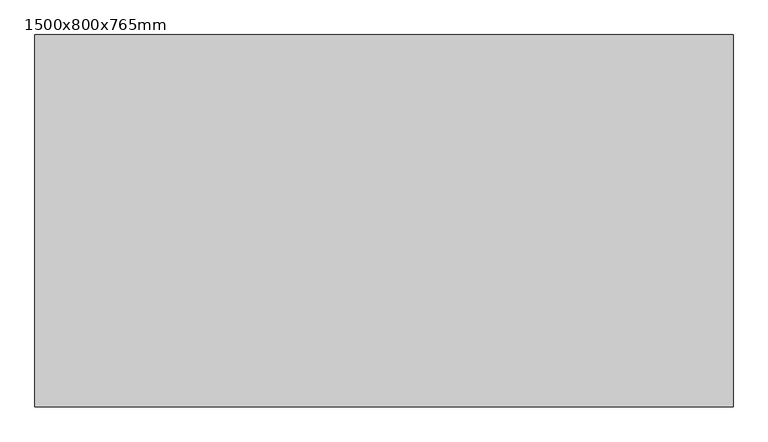
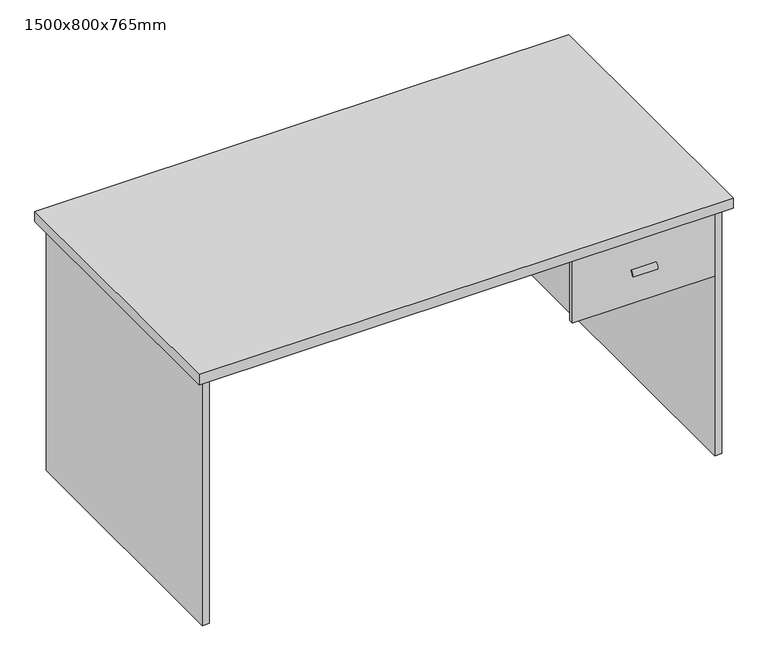
"""IFC4 building model written with IfcOpenShell, lengths in millimetres: furniture geometry, NBS_OffcDsks_OfficeDeskWithDrawer : 1500x800x765mm."""

import ifcopenshell
import ifcopenshell.guid

model = None  # the IFC model being written
_history = None  # IfcOwnerHistory: only IFC2X3 demands one
_inside = {}  # id of a spatial element -> (the spatial element, [elements in it])
_under = {}  # id of a project, library or spatial element -> (it, [spatial elements below it])
_declared = {}  # id of a project -> (the project, [libraries it declares])
_typed = {}  # id of a type object -> (the type object, [elements of that type])
_made_of = {}  # id of a material, layer set ... -> (it, [elements and type objects made of it])


def new_model(schema):
    """Start an empty IFC model of exactly this schema.

    Asked for "IFC4X3", IfcOpenShell would pick the latest addendum, in which some entities
    have other attributes; the version numbers below select the first issue.
    IFC2X3 requires an IfcOwnerHistory on every rooted entity: one is made here for all.
    """
    global model, _history
    if schema == "IFC4X3":
        model = ifcopenshell.file(schema_version=(4, 3, 0, 0))
    else:
        model = ifcopenshell.file(schema=schema)
    _inside.clear()
    _under.clear()
    _declared.clear()
    _typed.clear()
    _made_of.clear()
    _history = None
    if model.schema == "IFC2X3":
        org = make("IfcOrganization", Name="unknown")
        user = make(
            "IfcPersonAndOrganization",
            ThePerson=make("IfcPerson", FamilyName="unknown"),
            TheOrganization=org,
        )
        app = make(
            "IfcApplication",
            ApplicationDeveloper=org,
            Version="unknown",
            ApplicationFullName="unknown",
            ApplicationIdentifier="unknown",
        )
        _history = make(
            "IfcOwnerHistory",
            OwningUser=user,
            OwningApplication=app,
            ChangeAction="ADDED",
            CreationDate=0,
        )
    return model


def make(cls, **values):
    """One entity of the class cls with the attributes given. An attribute that is None is left unset."""
    return model.create_entity(
        cls, **{name: value for name, value in values.items() if value is not None}
    )


def rooted(cls, **values):
    """An entity with a GlobalId (a new one), such as an element, a storey or a relation."""
    return make(cls, GlobalId=ifcopenshell.guid.new(), OwnerHistory=_history, **values)


def si_unit(unit_type, name, prefix=None):
    """IfcSIUnit, for example si_unit("LENGTHUNIT", "METRE", prefix="MILLI")."""
    return make("IfcSIUnit", UnitType=unit_type, Prefix=prefix, Name=name)


def assignment(units):
    """IfcUnitAssignment: the units of a project."""
    return None if units is None else make("IfcUnitAssignment", Units=units)


def point(xyz):
    """IfcCartesianPoint."""
    return None if xyz is None else make("IfcCartesianPoint", Coordinates=xyz)


def direction(xyz):
    """IfcDirection."""
    return None if xyz is None else make("IfcDirection", DirectionRatios=xyz)


def frame(location, z_axis=None, x_axis=None):
    """IfcAxis2Placement3D, a coordinate frame: its origin and axes. An axis left out is left unset."""
    return make(
        "IfcAxis2Placement3D",
        Location=point(location),
        Axis=direction(z_axis),
        RefDirection=direction(x_axis),
    )


def frame_2d(location, x_axis=None):
    """IfcAxis2Placement2D, a coordinate frame in the plane: its origin and x axis."""
    return make(
        "IfcAxis2Placement2D", Location=point(location), RefDirection=direction(x_axis)
    )


def origin():
    """The frame at (0, 0, 0) with its axes left unset."""
    return frame((0.0, 0.0, 0.0))


def origin_with_axes():
    """The frame at (0, 0, 0) with the z axis (0, 0, 1) and the x axis (1, 0, 0) written out."""
    return frame((0.0, 0.0, 0.0), z_axis=(0.0, 0.0, 1.0), x_axis=(1.0, 0.0, 0.0))


def place(relative_to, where):
    """IfcLocalPlacement: puts the frame where relative to a parent placement (None: the world)."""
    return make(
        "IfcLocalPlacement", PlacementRelTo=relative_to, RelativePlacement=where
    )


def context(
    kind, dimensions, precision=None, world=None, true_north=None, identifier=None
):
    """IfcGeometricRepresentationContext, for example the 3D "Model" context."""
    return make(
        "IfcGeometricRepresentationContext",
        ContextIdentifier=identifier,
        ContextType=kind,
        CoordinateSpaceDimension=dimensions,
        Precision=precision,
        WorldCoordinateSystem=world,
        TrueNorth=true_north,
    )


def project(units=None, contexts=None):
    """IfcProject with its units and contexts."""
    return rooted(
        "IfcProject",
        Name="project",
        RepresentationContexts=contexts,
        UnitsInContext=assignment(units),
    )


def spatial(cls, under=None, at=None, **own):
    """A site, building, storey or space (cls), placed at a placement, below another one or the project."""
    s = rooted(cls, ObjectPlacement=at, **own)
    if under is not None:
        _under.setdefault(under.id(), (under, []))[1].append(s)
    return s


def polyline(points):
    """IfcPolyline through the points."""
    return make("IfcPolyline", Points=[point(p) for p in points])


def circle_curve(where, radius):
    """IfcCircle in the frame where."""
    return make("IfcCircle", Position=where, Radius=radius)


def trimmed(basis, trim1, trim2, sense, master):
    """IfcTrimmedCurve: the piece of a basis curve between two trims."""
    return make(
        "IfcTrimmedCurve",
        BasisCurve=basis,
        Trim1=trim1,
        Trim2=trim2,
        SenseAgreement=sense,
        MasterRepresentation=master,
    )


def segment(curve, same_sense, transition):
    """IfcCompositeCurveSegment."""
    return make(
        "IfcCompositeCurveSegment",
        Transition=transition,
        SameSense=same_sense,
        ParentCurve=curve,
    )


def composite_curve(segments, self_intersect=None):
    """IfcCompositeCurve: segments joined end to end."""
    return make("IfcCompositeCurve", Segments=segments, SelfIntersect=self_intersect)


def outline(outer, holes=None, kind="AREA"):
    """IfcArbitraryClosedProfileDef: a profile drawn as a closed curve; with holes, ...WithVoids."""
    if holes is None:
        return make("IfcArbitraryClosedProfileDef", ProfileType=kind, OuterCurve=outer)
    return make(
        "IfcArbitraryProfileDefWithVoids",
        ProfileType=kind,
        OuterCurve=outer,
        InnerCurves=holes,
    )


def extrude(swept, where, along, depth):
    """IfcExtrudedAreaSolid: the profile swept, set in the frame where, extruded along a direction by depth."""
    return make(
        "IfcExtrudedAreaSolid",
        SweptArea=swept,
        Position=where,
        ExtrudedDirection=direction(along),
        Depth=depth,
    )


def shape(context_of_items, identifier, shape_type, items):
    """IfcShapeRepresentation: the items that make up one representation, for example the "Body"."""
    return make(
        "IfcShapeRepresentation",
        ContextOfItems=context_of_items,
        RepresentationIdentifier=identifier,
        RepresentationType=shape_type,
        Items=items,
    )


def source(mapping_origin, context_of_items, identifier, shape_type, items):
    """IfcRepresentationMap: a shape defined once, which mapped items show again and again."""
    return make(
        "IfcRepresentationMap",
        MappingOrigin=mapping_origin,
        MappedRepresentation=shape(context_of_items, identifier, shape_type, items),
    )


def transform(
    local_origin,
    x_axis=None,
    y_axis=None,
    z_axis=None,
    scale=None,
    scale2=None,
    scale3=None,
    uniform=True,
):
    """IfcCartesianTransformationOperator3D, or its non-uniform kind. x_axis, y_axis, z_axis: its Axis1, 2, 3."""
    if uniform:
        return make(
            "IfcCartesianTransformationOperator3D",
            Axis1=direction(x_axis),
            Axis2=direction(y_axis),
            LocalOrigin=point(local_origin),
            Scale=scale,
            Axis3=direction(z_axis),
        )
    return make(
        "IfcCartesianTransformationOperator3DnonUniform",
        Axis1=direction(x_axis),
        Axis2=direction(y_axis),
        LocalOrigin=point(local_origin),
        Scale=scale,
        Axis3=direction(z_axis),
        Scale2=scale2,
        Scale3=scale3,
    )


def mapped(mapping_source, mapping_target):
    """IfcMappedItem: shows the shape of a source again, moved by a transform."""
    return make(
        "IfcMappedItem", MappingSource=mapping_source, MappingTarget=mapping_target
    )


def made_of(thing, what):
    """Note that an element or type object is made of a material, layer set ...; save() writes the relation."""
    if what is not None:
        _made_of.setdefault(what.id(), (what, []))[1].append(thing)
    return thing


def element(
    cls,
    number,
    at=None,
    inside=None,
    cuts=None,
    type_object=None,
    material=None,
    context=None,
    identifier="Body",
    shape_type=None,
    held_by="IfcProductDefinitionShape",
    body=None,
    shapes=None,
    **own,
):
    """One element of the class cls, such as IfcWall. Its Tag is "e" and its number.

    at: its placement. inside: the storey or other place that contains it. cuts: it is an
    opening in that element (IfcRelVoidsElement). A single representation is given by context,
    identifier, shape_type and body (its items); several are given by shapes. held_by: the class
    of the entity that holds the representations. save() writes the other relations.
    """
    e = rooted(cls, Tag="e%d" % number, ObjectPlacement=at, **own)
    if body is not None:
        shapes = [shape(context, identifier, shape_type, body)]
    if shapes is not None:
        e.Representation = make(held_by, Representations=shapes)
    if inside is not None:
        _inside.setdefault(inside.id(), (inside, []))[1].append(e)
    if cuts is not None:
        rooted(
            "IfcRelVoidsElement", RelatingBuildingElement=cuts, RelatedOpeningElement=e
        )
    if type_object is not None:
        _typed.setdefault(type_object.id(), (type_object, []))[1].append(e)
    return made_of(e, material)


def aggregate(whole, parts):
    """IfcRelAggregates: a whole, such as a stair, and the parts it consists of."""
    return rooted("IfcRelAggregates", RelatingObject=whole, RelatedObjects=parts)


def save(model, path):
    """Write the relations noted so far, then the file.

    IfcRelAggregates (storeys below a building ...), IfcRelContainedInSpatialStructure (elements
    in a storey), IfcRelDefinesByType, IfcRelAssociatesMaterial and IfcRelDeclares: one each for
    every whole, place, type object, material and project.
    """
    for whole, parts in _under.values():
        aggregate(whole, parts)
    for where, things in _inside.values():
        rooted(
            "IfcRelContainedInSpatialStructure",
            RelatedElements=things,
            RelatingStructure=where,
        )
    for kind, things in _typed.values():
        rooted("IfcRelDefinesByType", RelatedObjects=things, RelatingType=kind)
    for what, things in _made_of.values():
        rooted("IfcRelAssociatesMaterial", RelatedObjects=things, RelatingMaterial=what)
    for by, libraries in _declared.values():
        rooted("IfcRelDeclares", RelatingContext=by, RelatedDefinitions=libraries)
    model.write(path)


def furniture_1500x800x765mm_9c7e9ddd(model_context):
    return source(origin(), model_context, "Body", "SweptSolid", [
        extrude(outline(polyline([(710.0, -380.0), (310.0, -380.0), (310.0, -368.0), (710.0, -368.0), (710.0, -380.0)])), frame((0.0, 0.0, 535.0), z_axis=(0.0, 0.0, 1.0), x_axis=(1.0, 0.0, 0.0)), (0.0, 0.0, 1.0), 200.0),
        extrude(outline(polyline([(698.0, 60.0), (698.0, -368.0), (321.9992987, -368.0), (321.9992987, 60.0), (698.0, 60.0)])), frame((0.0, 0.0, 540.7416159), z_axis=(0.0, 0.0, 1.0), x_axis=(1.0, 0.0, 0.0)), (0.0, 0.0, 1.0), 194.2583841),
        extrude(outline(polyline([(710.0, 380.0), (710.0, 360.0), (-710.0, 360.0), (-710.0, 380.0), (710.0, 380.0)])), frame((0.0, 0.0, 185.0), z_axis=(0.0, 0.0, 1.0), x_axis=(1.0, 0.0, 0.0)), (0.0, 0.0, 1.0), 550.0),
        extrude(outline(polyline([(-710.0, 380.0), (-710.0, -380.0), (-730.0, -380.0), (-730.0, 380.0), (-710.0, 380.0)])), origin_with_axes(), (0.0, 0.0, 1.0), 735.0),
        extrude(outline(polyline([(730.0, 380.0), (730.0, -380.0), (710.0, -380.0), (710.0, 380.0), (730.0, 380.0)])), origin_with_axes(), (0.0, 0.0, 1.0), 735.0),
        extrude(outline(polyline([(750.0, 400.0), (750.0, -400.0), (-750.0, -400.0), (-750.0, 400.0), (750.0, 400.0)])), frame((0.0, 0.0, 735.0), z_axis=(0.0, 0.0, 1.0), x_axis=(1.0, 0.0, 0.0)), (0.0, 0.0, 1.0), 30.0),
        extrude(outline(composite_curve([segment(trimmed(circle_curve(frame_2d((-369.1756558, 618.6602663)), 20.2222385), [point((-389.3776536, 619.5648197))], [point((-380.0, 635.7416159))], False, "CARTESIAN"), True, "CONTINUOUS"), segment(polyline([(-380.0, 635.7416159), (-380.0, 631.5709177)]), True, "CONTINUOUS"), segment(trimmed(circle_curve(frame_2d((-367.0301873, 617.1513707)), 19.394313), [point((-380.0, 631.5709177))], [point((-384.452251, 625.6725838))], True, "CARTESIAN"), True, "CONTINUOUS"), segment(trimmed(circle_curve(frame_2d((-393.0621605, 627.5759127)), 8.8177776), [point((-384.452251, 625.6725838))], [point((-389.3776536, 619.5648197))], False, "CARTESIAN"), True, "CONTINUOUS")], self_intersect=False)), frame((475.0, 0.0, 0.0), z_axis=(1.0, 0.0, 0.0), x_axis=(0.0, 1.0, 0.0)), (0.0, 0.0, 1.0), 70.0),
    ])


if __name__ == "__main__":
    model = new_model("IFC4")
    model_context = context("Model", 3, world=origin())
    ifc_project = project(units=[si_unit("LENGTHUNIT", "METRE", prefix="MILLI")], contexts=[model_context])
    site = spatial("IfcSite", under=ifc_project)
    building = spatial("IfcBuilding", under=site)
    placement = place(None, origin())
    furniture_1500x800x765mm_shape = furniture_1500x800x765mm_9c7e9ddd(model_context)
    element("IfcFurniture", 1, ObjectType="NBS_OffcDsks_OfficeDeskWithDrawer : 1500x800x765mm", at=placement, inside=building, context=model_context, shape_type="MappedRepresentation", body=[
        mapped(furniture_1500x800x765mm_shape, transform((0.0, 0.0, 0.0), x_axis=(1.0, 0.0, 0.0), y_axis=(0.0, 1.0, 0.0), z_axis=(0.0, 0.0, 1.0))),
    ])
    save(model, "model.ifc")

# Revit data of these elements
# Project information
#   Projekt-Nummer = "Hier die Projektnummer eintragen!"
#   IfcSite GUID = "3DdyCULLv3kQRx$MQ8PThJ"
#   IfcBuilding GUID = "3DdyCULLv3kQRx$MQ8PThG"
#   IfcProject GUID = "3DdyCULLv3kQRx$MQ8PThH"
#   Classification.Facility.Number = "Co_20_15_58"
#   Classification.Facility.Description = "Office complexes"
#   Project Status = "Projektstatus"
#   Project Address = "Geben Sie die Adresse hier ein"
# Type "NBS_OffcDsks_OfficeDeskWithDrawer : 1500x800x765mm"
#   Type IfcGUID = "2u0XNFrAPALBFZCv81fq27"
#   WarrantyStartDate [instance default] = "1900-12-31T23:59:59"
#   WarrantyGuarantorParts = "n/a"
#   WarrantyGuarantorLabor = "n/a"
#   WarrantyDurationUnit = "year"
#   WarrantyDurationParts = "n/a"
#   WarrantyDurationLabor = "n/a"
#   WarrantyDescription = "n/a"
#   Version = "2"
#   Uniclass2015Version = "Products v1.9"
#   Uniclass2015Title = "Office desks"
#   Uniclass2015Code = "Pr_40_50_21_59"
#   URL = "www.nationalbimlibrary.com"
#   TagNumber [instance default] = "n/a"
#   SustainabilityPerformance = "n/a"
#   Style = "n/a"
#   Size = "1500 x 800 x 765 mm"
#   Shape = "n/a"
#   SerialNumber [instance default] = "n/a"
#   Revision = "n/a"
#   ReplacementCost = "n/a"
#   ProductInformation = "www.nationalbimlibrary.com"
#   OmniClassVersion = "Table 22 2012-05-16"
#   OmniClassTitle = "Office Tables"
#   OmniClassCode = "22-12 51 23"
#   Name = "OfficeDesks_OfficeDeskWithDrawer"
#   NBSReference = "45-35-20/335"
#   NBSDescription = "Office desks"
#   NBSCertification = "www.nationalbimlibrary.com/cert/b4qdjtam"
#   ModelReference = "Office Desk with Drawer"
#   ModelNumber = "n/a"
#   Model = "Office Desk with Drawer"
#   Material = "n/a"
#   ManufacturerURL = "n/a"
#   ManufacturerName = "n/a"
#   Manufacturer = "info@theNBS.com"
#   MainColor = "n/a"
#   InstallationDate [instance default] = "1900-12-31T23:59:59"
#   IfcExportType = "DESK"
#   IfcExportAs = "IfcFurnitureType"
#   Grade = "n/a"
#   Finish = "n/a"
#   Features = "n/a"
#   ExpectedLife = "n/a"
#   DurationUnit = "year"
#   Description = "Generic rectangular office desk with drawer"
#   Constituents = "n/a"
#   Color = "n/a"
#   CodePerformance = "n/a"
#   Category = "Pr_40_50_21_59:Office desks"
#   BarCode [instance default] = "n/a"
#   BIMObjectName = "NBS_OfficeDesks_OfficeDeskWithDrawer"
#   Author = "NBS"
#   AssetType = "Movable"
#   AssetIdentifier [instance default] = "n/a"
#   AccessibilityPerformance = "n/a"
#   WorksurfaceArea = 104.051405 m²
#   NominalWidth = 0.8 m
#   NominalHeight = 0.765 m
#   DesktopThickness = 0.03 m
#   NominalLength = 1.5 m
#   NominalDepth = 0.8 m
#   DrawerFaceWidth = 0.4 m
#   DrawerFaceHeight = 0.2 m
#   DeskLegThickness = 0.02 m
#   DeskLegOffset = 0.02 m
#   DrawerLength = 0.44 m
#   DeskBackDrop = 0.55 m
#   HandleMaterial = NBS_Concept
#   DrawerMaterial = NBS_Concept
#   DesktopMaterial = NBS_Concept
#   DeskSupportMaterial = NBS_Concept
#   Default Elevation = 0
#   Cost = 0
# Element 1 (IfcFurniture, "NBS_OffcDsks_OfficeDeskWithDrawer : 1500x800x765mm")
#   Materials on its faces: "NBS_Concept"
# Materials
#   "NBS_Concept": class "Generic", colour RGB 255 255 255, transparency 0, Description = "To be specified", Cost = 0
